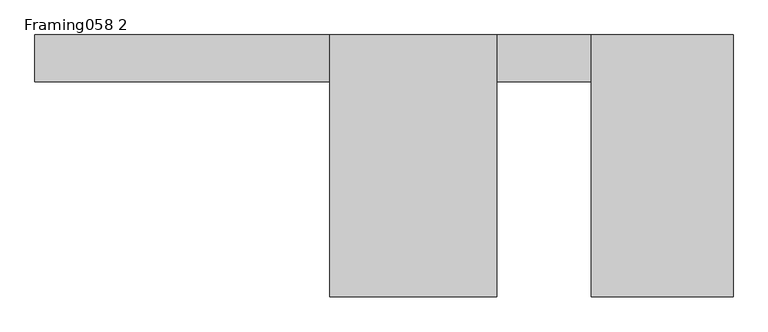
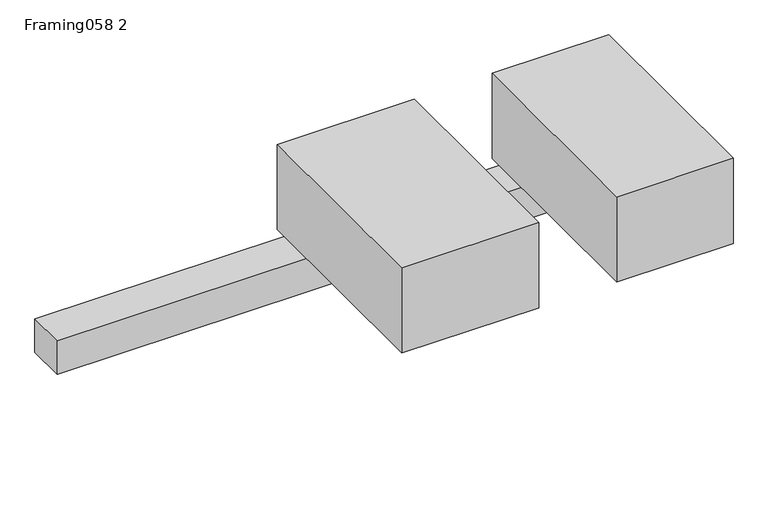
"""IFC4 building model written with IfcOpenShell, lengths in millimetres: proxy geometry, Framing058 2 : Framing058 14884."""

from ifc_helpers import new_model, si_unit, frame, origin, place, context, project, spatial, polyline, outline, extrude, source, transform, mapped, element, save


def framing058_2_ada2c0c3(model_context):
    return source(origin(), model_context, "Body", "SweptSolid", [
        extrude(outline(polyline([(-429.5688412, 96.9874752), (-889.0664422, 96.9874752), (-889.0664422, 947.1093426), (-429.5688412, 947.1093426), (-429.5688412, 96.9874752)])), frame((0.0, 0.0, 39757.096), z_axis=(0.0, 0.0, 1.0), x_axis=(1.0, 0.0, 0.0)), (0.0, 0.0, 1.0), 355.6),
        extrude(outline(polyline([(-1196.4064422, 96.9874752), (-1738.0614422, 96.9874752), (-1738.0614422, 947.1093426), (-1196.4064422, 947.1093426), (-1196.4064422, 96.9874752)])), frame((0.0, 0.0, 39757.096), z_axis=(0.0, 0.0, 1.0), x_axis=(1.0, 0.0, 0.0)), (0.0, 0.0, 1.0), 355.6),
        extrude(outline(polyline([(-718.8864422, 794.7093426), (-2694.3737014, 794.7093426), (-2694.3737014, 947.1093426), (-718.8864422, 947.1093426), (-718.8864422, 794.7093426)])), frame((0.0, 0.0, 39579.2960083), z_axis=(0.0, 0.0, 1.0), x_axis=(1.0, 0.0, 0.0)), (0.0, 0.0, 1.0), 139.7),
    ])


if __name__ == "__main__":
    model = new_model("IFC4")
    model_context = context("Model", 3, world=origin())
    ifc_project = project(units=[si_unit("LENGTHUNIT", "METRE", prefix="MILLI")], contexts=[model_context])
    site = spatial("IfcSite", under=ifc_project)
    building = spatial("IfcBuilding", under=site)
    placement = place(None, origin())
    framing058_2_shape = framing058_2_ada2c0c3(model_context)
    element("IfcBuildingElementProxy", 1, Name="Framing058 2 : Framing058 14884", ObjectType="Framing058 2 : Framing058 14884", at=placement, inside=building, context=model_context, shape_type="MappedRepresentation", body=[
        mapped(framing058_2_shape, transform((0.0, 0.0, 0.0), x_axis=(1.0, 0.0, 0.0), y_axis=(0.0, 1.0, 0.0), z_axis=(0.0, 0.0, 1.0))),
    ])
    save(model, "model.ifc")

# Revit data of these elements
# Type "Framing058 2 : Framing058 14884"
#   NameOverride = "Framing058"
# Element 1 (IfcBuildingElementProxy, "Framing058 2 : Framing058 14884")
#   Materials on its faces: "WOOD FRAMING (SEE STRUCT DWGS)"
# Materials
#   "WOOD FRAMING (SEE STRUCT DWGS)": class "Unassigned", colour RGB 224 188 168, transparency 0, Cost = 0
